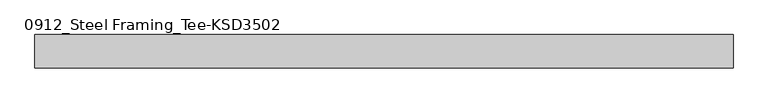
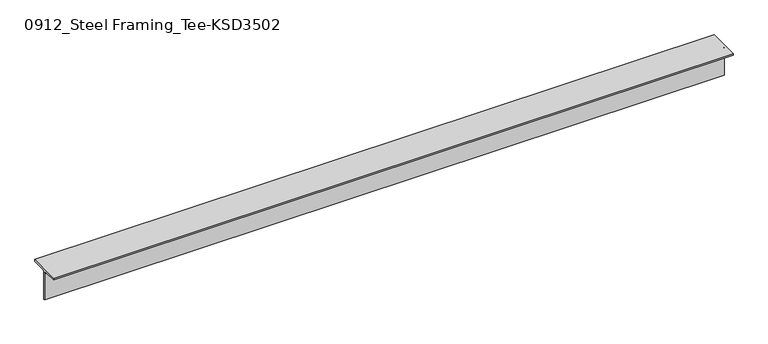
"""IFC4 building model written with IfcOpenShell, lengths in millimetres: member geometry, 0912_Steel Framing_Tee-KSD3502 : H_SB_ASB_CT-150x150x6.5x9."""

from ifc_helpers import new_model, si_unit, point, frame, frame_2d, origin, place, context, project, spatial, polyline, circle_curve, trimmed, segment, composite_curve, outline, extrude, source, transform, mapped, element, save


def member_0912_steel_framing_tee_ksd3502_04e40f12(model_context):
    return source(origin(), model_context, "Body", "SweptSolid", [
        extrude(outline(composite_curve([segment(polyline([(-75.0, 75.0), (75.0, 75.0), (75.0, 66.0), (16.25, 66.0)]), True, "CONTINUOUS"), segment(trimmed(circle_curve(frame_2d((16.25, 53.0)), 13.0), [point((16.25, 66.0))], [point((3.25, 53.0))], True, "CARTESIAN"), True, "CONTINUOUS"), segment(polyline([(3.25, 53.0), (3.25, -75.0), (-3.25, -75.0), (-3.25, 53.0)]), True, "CONTINUOUS"), segment(trimmed(circle_curve(frame_2d((-16.25, 53.0)), 13.0), [point((-3.25, 53.0))], [point((-16.25, 66.0))], True, "CARTESIAN"), True, "CONTINUOUS"), segment(polyline([(-16.25, 66.0), (-75.0, 66.0), (-75.0, 75.0)]), True, "CONTINUOUS")], self_intersect=False)), frame((-1617.1, 0.0, 0.0), z_axis=(1.0, 0.0, 0.0), x_axis=(0.0, 1.0, 0.0)), (0.0, 0.0, 1.0), 3133.1),
    ])


if __name__ == "__main__":
    model = new_model("IFC4")
    model_context = context("Model", 3, world=origin())
    ifc_project = project(units=[si_unit("LENGTHUNIT", "METRE", prefix="MILLI")], contexts=[model_context])
    site = spatial("IfcSite", under=ifc_project)
    building = spatial("IfcBuilding", under=site)
    placement = place(None, origin())
    member_0912_steel_framing_tee_ksd3502_shape = member_0912_steel_framing_tee_ksd3502_04e40f12(model_context)
    element("IfcMember", 1, ObjectType="0912_Steel Framing_Tee-KSD3502 : H_SB_ASB_CT-150x150x6.5x9", at=placement, inside=building, context=model_context, shape_type="MappedRepresentation", body=[
        mapped(member_0912_steel_framing_tee_ksd3502_shape, transform((0.0, 0.0, 0.0), x_axis=(1.0, 0.0, 0.0), y_axis=(0.0, 1.0, 0.0), z_axis=(0.0, 0.0, 1.0))),
    ])
    save(model, "model.ifc")

# Revit data of these elements
# Type "0912_Steel Framing_Tee-KSD3502 : H_SB_ASB_CT-150x150x6.5x9"
#   H_WM Code_1 = "S01AA003-00001 | Main Steel Structure Fabrication Work | Shelter/Building | Light Steel - Standard (30KG/M>Weight) | Material: (   )"
#   H_WM Code_2 = "S03AA029-00001 | Main Steel Structure Erection Work | Shelter/Building | Light Steel (30KG/M>Weight) | Material: (   )"
#   H_WM Code_3 = "S01AA010-00001 | Main Steel Structure Fabrication Work | Shelter/Building | Steel Painting/Coating | for Non-Fireproofed Steel Surface, Surface Preparation, Primer, Second & Final Coat | Material: (   )"
#   H_Q'ty Cal Type Tag = "SB-Q2"
#   Width = 15.0 cm
#   Web Thickness = 0.65 cm
#   Web Fillet = 1.3 cm
#   Section Area = 23.39 cm²
#   Perimeter = 0.60 m²/m
#   Nominal Weight = 18.40 kgf/m
#   Height = 15.0 cm
#   Flange Thickness = 0.9 cm
#   Centroid Vertical = 7.5 cm
#   Centroid Horizontal = 7.5 cm
#   Length [instance default] = 1.5000 m
#   Structural Material [instance default] = Steel, 45-345
#   Warping Constant = (empty or 0)
#   Torsional Moment of Inertia = 0
#   Section Name Key = ""
#   Plastic Modulus weak axis = 0
#   Plastic Modulus strong axis = 0
#   Moment of Inertia weak axis = 0
#   Moment of Inertia strong axis = 0
#   Elastic Modulus weak axis = 0
#   Elastic Modulus strong axis = 0
#   Bolt Spacing = 0
#   Assembly Code = ""
# Element 1 (IfcMember, "0912_Steel Framing_Tee-KSD3502 : H_SB_ASB_CT-150x150x6.5x9")
#   Structural Material = none
# Materials
#   "Steel, 45-345": class "Metal", colour RGB 189 187 185, transparency 0, Description = "Steel 345 MPa", Cost = 0
